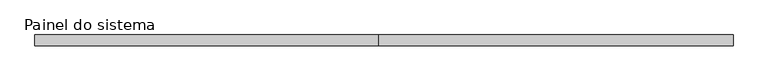
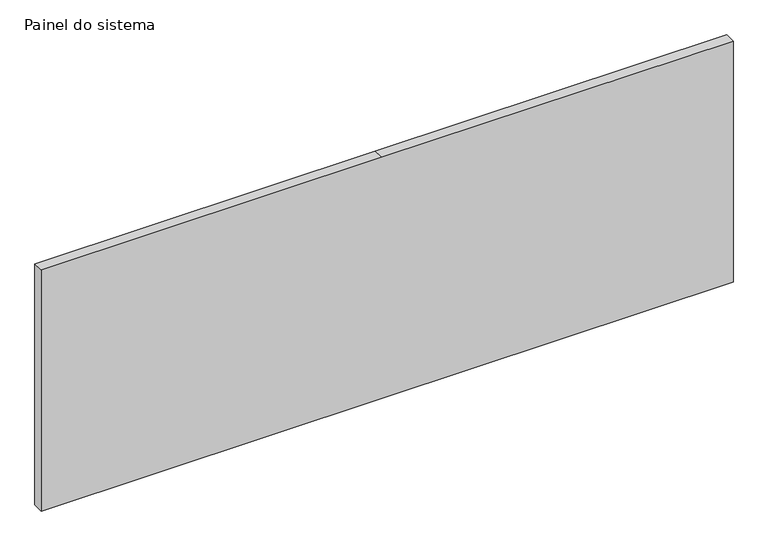
"""IFC4 building model written with IfcOpenShell, lengths in millimetres: plate geometry, Painel do sistema : Envidraçado."""

from ifc_helpers import new_model, si_unit, frame, origin, place, context, project, spatial, polyline, outline, extrude, source, transform, mapped, element, save


def painel_do_sistema_304b63e8(model_context):
    return source(origin(), model_context, "Body", "SweptSolid", [
        extrude(outline(polyline([(0.0, -800.0500001), (0.0, -12.4999998), (0.0, 800.0500001), (590.0, 800.0500001), (590.0, -12.4999998), (590.0, -800.0500001), (0.0, -800.0500001)])), frame((0.0, -49.5, 0.0), z_axis=(0.0, 1.0, 0.0), x_axis=(0.0, 0.0, 1.0)), (0.0, 0.0, 1.0), 25.0),
    ])


if __name__ == "__main__":
    model = new_model("IFC4")
    model_context = context("Model", 3, world=origin())
    ifc_project = project(units=[si_unit("LENGTHUNIT", "METRE", prefix="MILLI")], contexts=[model_context])
    site = spatial("IfcSite", under=ifc_project)
    building = spatial("IfcBuilding", under=site)
    placement = place(None, origin())
    painel_do_sistema_shape = painel_do_sistema_304b63e8(model_context)
    element("IfcPlate", 1, ObjectType="Painel do sistema : Envidraçado", at=placement, inside=building, context=model_context, shape_type="MappedRepresentation", body=[
        mapped(painel_do_sistema_shape, transform((0.0, 0.0, 0.0), x_axis=(1.0, 0.0, 0.0), y_axis=(0.0, 1.0, 0.0), z_axis=(0.0, 0.0, 1.0))),
    ])
    save(model, "model.ifc")

# Revit data of these elements
# Type "Painel do sistema : Envidraçado"
#   Construction Type Id = "GSP4R"
#   Analytic Construction = "Vidraça única Pilkington 1/8 pol"
#   Visual Light Transmittance = 0.9
#   Solar Heat Gain Coefficient = 0.86
#   Heat Transfer Coefficient (U) = 6.7069 W/(m²·K)
# Element 1 (IfcPlate, "Painel do sistema : Envidraçado")
#   Materials on its faces: ".VIDRO GENÉRICO"
# Materials
#   ".VIDRO GENÉRICO": class ".CC_VIDRO", colour RGB 0 128 192, transparency 0.9, Description = "Vidro comum", Cost = 0
